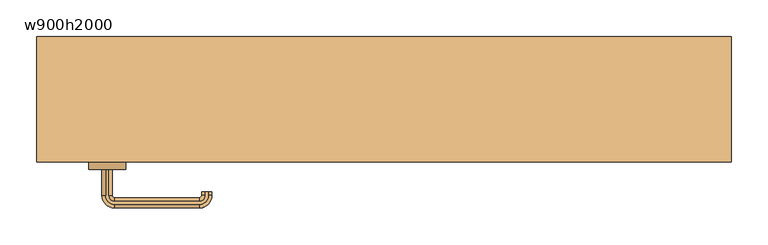
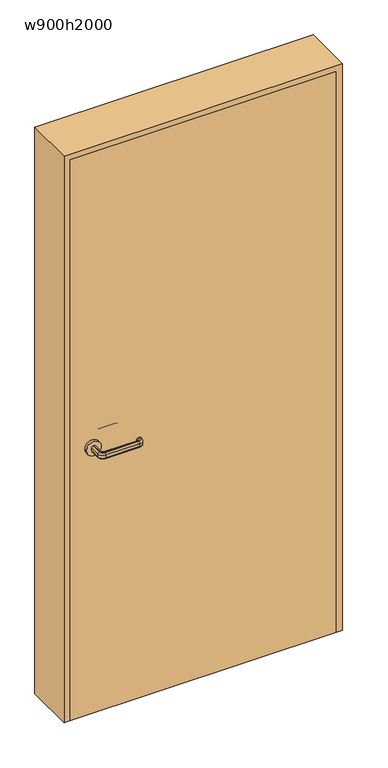
"""IFC4 building model written with IfcOpenShell, lengths in millimetres: door geometry, 片開き : w900h2000."""

from ifc_helpers import new_model, si_unit, point, frame, frame_2d, origin, origin_with_axes, place, context, project, spatial, polyline, circle_curve, ellipse_curve, trimmed, segment, composite_curve, outline, extrude, source, transform, mapped, element, save
from ifc_brep_helpers import plane_surface, cylinder_surface, revolved_surface, advanced_brep


def w900h2000_c063673d(model_context):
    return source(origin(), model_context, "Body", "SolidModel", [
        advanced_brep(
        [(-377.0, -95.0, 960.0), (-373.0, -95.0, 960.0), (-368.0, -95.0, 955.0), (-368.0, -95.0, 945.0477623), (-373.0, -95.0, 940.0477623), (-377.0, -95.0, 940.0477623), (-382.0, -95.0, 945.0477623), (-382.0, -95.0, 955.0), (-382.0, -130.0, 955.0), (-377.0, -130.0, 960.0), (-382.0, -130.0, 945.0477623), (-377.0, -130.0, 940.0477623), (-373.0, -130.0, 940.0477623), (-365.0, -138.0, 940.0477623), (-250.0, -138.0, 940.0477623), (-242.0, -130.0, 940.0477623), (-242.0, -125.0, 940.0477623), (-238.0, -125.0, 940.0477623), (-238.0, -130.0, 940.0477623), (-250.0, -142.0, 940.0477623), (-365.0, -142.0, 940.0477623), (-368.0, -130.0, 945.0477623), (-368.0, -130.0, 955.0), (-373.0, -130.0, 960.0), (-365.0, -142.0, 960.0), (-250.0, -142.0, 960.0), (-238.0, -130.0, 960.0), (-238.0, -125.0, 960.0), (-242.0, -125.0, 960.0), (-242.0, -130.0, 960.0), (-250.0, -138.0, 960.0), (-365.0, -138.0, 960.0), (-365.0, -147.0, 955.0), (-365.0, -147.0, 945.0477623), (-365.0, -133.0, 945.0477623), (-365.0, -133.0, 955.0), (-250.0, -147.0, 955.0), (-250.0, -147.0, 945.0477623), (-250.0, -133.0, 945.0477623), (-250.0, -133.0, 955.0), (-233.0, -130.0, 955.0), (-233.0, -130.0, 945.0477623), (-247.0, -130.0, 945.0477623), (-247.0, -130.0, 955.0), (-233.0, -125.0, 955.0), (-233.0, -125.0, 945.0477623), (-247.0, -125.0, 945.0477623), (-247.0, -125.0, 955.0)],
        [
            (0, 1),
            (1, 2, circle_curve(frame((-373.0, -95.0, 955.0), z_axis=(0.0, 1.0, 0.0), x_axis=(-1.0, 0.0, 0.0)), 5.0)),
            (2, 3),
            (3, 4, circle_curve(frame((-373.0, -95.0, 945.0477623), z_axis=(0.0, 1.0, 0.0), x_axis=(-1.0, 0.0, 0.0)), 5.0)),
            (4, 5),
            (5, 6, circle_curve(frame((-377.0, -95.0, 945.0477623), z_axis=(0.0, 1.0, 0.0), x_axis=(-1.0, 0.0, 0.0)), 5.0)),
            (6, 7),
            (7, 0, circle_curve(frame((-377.0, -95.0, 955.0), z_axis=(0.0, 1.0, 0.0), x_axis=(-1.0, 0.0, 0.0)), 5.0)),
            (7, 8),
            (8, 9, circle_curve(frame((-377.0, -130.0, 955.0), z_axis=(0.0, 1.0, 0.0), x_axis=(-1.0, 0.0, 0.0)), 5.0)),
            (9, 0),
            (6, 10),
            (10, 8),
            (5, 11),
            (11, 10, circle_curve(frame((-377.0, -130.0, 945.0477623), z_axis=(0.0, 1.0, 0.0), x_axis=(-1.0, 0.0, 0.0)), 5.0)),
            (4, 12),
            (12, 13, circle_curve(frame((-365.0, -130.0, 940.0477623), z_axis=(0.0, 0.0, 1.0), x_axis=(-1.0, 0.0, 0.0)), 8.0)),
            (13, 14),
            (14, 15, circle_curve(frame((-250.0, -130.0, 940.0477623), z_axis=(0.0, 0.0, 1.0), x_axis=(0.0, -1.0, 0.0)), 8.0)),
            (15, 16),
            (16, 17),
            (17, 18),
            (18, 19, circle_curve(frame((-250.0, -130.0, 940.0477623), z_axis=(0.0, 0.0, -1.0), x_axis=(0.0, -1.0, 0.0)), 12.0)),
            (19, 20),
            (20, 11, circle_curve(frame((-365.0, -130.0, 940.0477623), z_axis=(0.0, 0.0, -1.0), x_axis=(-1.0, 0.0, 0.0)), 12.0)),
            (3, 21),
            (21, 12, circle_curve(frame((-373.0, -130.0, 945.0477623), z_axis=(0.0, 1.0, 0.0), x_axis=(-1.0, 0.0, 0.0)), 5.0)),
            (2, 22),
            (22, 21),
            (1, 23),
            (23, 22, circle_curve(frame((-373.0, -130.0, 955.0), z_axis=(0.0, 1.0, 0.0), x_axis=(-1.0, 0.0, 0.0)), 5.0)),
            (9, 24, circle_curve(frame((-365.0, -130.0, 960.0), z_axis=(0.0, 0.0, 1.0), x_axis=(-1.0, 0.0, 0.0)), 12.0)),
            (24, 25),
            (25, 26, circle_curve(frame((-250.0, -130.0, 960.0), z_axis=(0.0, 0.0, 1.0), x_axis=(0.0, -1.0, 0.0)), 12.0)),
            (26, 27),
            (27, 28),
            (28, 29),
            (29, 30, circle_curve(frame((-250.0, -130.0, 960.0), z_axis=(0.0, 0.0, -1.0), x_axis=(0.0, -1.0, 0.0)), 8.0)),
            (30, 31),
            (31, 23, circle_curve(frame((-365.0, -130.0, 960.0), z_axis=(0.0, 0.0, -1.0), x_axis=(-1.0, 0.0, 0.0)), 8.0)),
            (32, 24, circle_curve(frame((-365.0, -142.0, 955.0), z_axis=(-1.0, 0.0, 0.0), x_axis=(0.0, -1.0, 0.0)), 5.0)),
            (8, 32, circle_curve(frame((-365.0, -130.0, 955.0), z_axis=(0.0, 0.0, 1.0), x_axis=(-1.0, 0.0, 0.0)), 17.0)),
            (33, 32),
            (10, 33, circle_curve(frame((-365.0, -130.0, 945.0477623), z_axis=(0.0, 0.0, 1.0), x_axis=(-1.0, 0.0, 0.0)), 17.0)),
            (20, 33, circle_curve(frame((-365.0, -142.0, 945.0477623), z_axis=(-1.0, 0.0, 0.0), x_axis=(0.0, -1.0, 0.0)), 5.0)),
            (34, 13, circle_curve(frame((-365.0, -138.0, 945.0477623), z_axis=(-1.0, 0.0, 0.0), x_axis=(0.0, -1.0, 0.0)), 5.0)),
            (21, 34, circle_curve(frame((-365.0, -130.0, 945.0477623), z_axis=(0.0, 0.0, 1.0), x_axis=(-1.0, 0.0, 0.0)), 3.0)),
            (35, 34),
            (22, 35, circle_curve(frame((-365.0, -130.0, 955.0), z_axis=(0.0, 0.0, 1.0), x_axis=(-1.0, 0.0, 0.0)), 3.0)),
            (31, 35, circle_curve(frame((-365.0, -138.0, 955.0), z_axis=(-1.0, 0.0, 0.0), x_axis=(0.0, -1.0, 0.0)), 5.0)),
            (32, 36),
            (36, 25, circle_curve(frame((-250.0, -142.0, 955.0), z_axis=(-1.0, 0.0, 0.0), x_axis=(0.0, -1.0, 0.0)), 5.0)),
            (33, 37),
            (37, 36),
            (19, 37, circle_curve(frame((-250.0, -142.0, 945.0477623), z_axis=(-1.0, 0.0, 0.0), x_axis=(0.0, -1.0, 0.0)), 5.0)),
            (34, 38),
            (38, 14, circle_curve(frame((-250.0, -138.0, 945.0477623), z_axis=(-1.0, 0.0, 0.0), x_axis=(0.0, -1.0, 0.0)), 5.0)),
            (35, 39),
            (39, 38),
            (30, 39, circle_curve(frame((-250.0, -138.0, 955.0), z_axis=(-1.0, 0.0, 0.0), x_axis=(0.0, -1.0, 0.0)), 5.0)),
            (40, 26, circle_curve(frame((-238.0, -130.0, 955.0), z_axis=(0.0, -1.0, 0.0), x_axis=(1.0, 0.0, 0.0)), 5.0)),
            (36, 40, circle_curve(frame((-250.0, -130.0, 955.0), z_axis=(0.0, 0.0, 1.0), x_axis=(0.0, -1.0, 0.0)), 17.0)),
            (41, 40),
            (37, 41, circle_curve(frame((-250.0, -130.0, 945.0477623), z_axis=(0.0, 0.0, 1.0), x_axis=(0.0, -1.0, 0.0)), 17.0)),
            (18, 41, circle_curve(frame((-238.0, -130.0, 945.0477623), z_axis=(0.0, -1.0, 0.0), x_axis=(1.0, 0.0, 0.0)), 5.0)),
            (42, 15, circle_curve(frame((-242.0, -130.0, 945.0477623), z_axis=(0.0, -1.0, 0.0), x_axis=(1.0, 0.0, 0.0)), 5.0)),
            (38, 42, circle_curve(frame((-250.0, -130.0, 945.0477623), z_axis=(0.0, 0.0, 1.0), x_axis=(0.0, -1.0, 0.0)), 3.0)),
            (43, 42),
            (39, 43, circle_curve(frame((-250.0, -130.0, 955.0), z_axis=(0.0, 0.0, 1.0), x_axis=(0.0, -1.0, 0.0)), 3.0)),
            (29, 43, circle_curve(frame((-242.0, -130.0, 955.0), z_axis=(0.0, -1.0, 0.0), x_axis=(1.0, 0.0, 0.0)), 5.0)),
            (27, 44, circle_curve(frame((-238.0, -125.0, 955.0), z_axis=(0.0, 1.0, 0.0), x_axis=(1.0, 0.0, 0.0)), 5.0)),
            (44, 45),
            (45, 17, circle_curve(frame((-238.0, -125.0, 945.0477623), z_axis=(0.0, 1.0, 0.0), x_axis=(1.0, 0.0, 0.0)), 5.0)),
            (16, 46, circle_curve(frame((-242.0, -125.0, 945.0477623), z_axis=(0.0, 1.0, 0.0), x_axis=(1.0, 0.0, 0.0)), 5.0)),
            (46, 47),
            (47, 28, circle_curve(frame((-242.0, -125.0, 955.0), z_axis=(0.0, 1.0, 0.0), x_axis=(1.0, 0.0, 0.0)), 5.0)),
            (40, 44),
            (41, 45),
            (42, 46),
            (43, 47),
        ],
        [
            plane_surface(frame((-385.198039, -95.0, 950.0), z_axis=(0.0, 1.0, 0.0), x_axis=(0.0, 0.0, 1.0))),
            cylinder_surface(frame((-377.0, -95.0, 955.0), z_axis=(0.0, 1.0, 0.0), x_axis=(-1.0, 0.0, 0.0)), 5.0),
            plane_surface(frame((-382.0, -95.0, 955.0), z_axis=(-1.0, 0.0, 0.0), x_axis=(0.0, -1.0, 0.0))),
            cylinder_surface(frame((-377.0, -95.0, 945.0477623), z_axis=(0.0, 1.0, 0.0), x_axis=(-1.0, 0.0, 0.0)), 5.0),
            plane_surface(frame((-377.0, -95.0, 940.0477623), z_axis=(0.0, 0.0, -1.0), x_axis=(0.0, -1.0, 0.0))),
            cylinder_surface(frame((-373.0, -95.0, 945.0477623), z_axis=(0.0, 1.0, 0.0), x_axis=(-1.0, 0.0, 0.0)), 5.0),
            plane_surface(frame((-368.0, -95.0, 945.0477623), z_axis=(1.0, 0.0, 0.0), x_axis=(0.0, -1.0, 0.0))),
            cylinder_surface(frame((-373.0, -95.0, 955.0), z_axis=(0.0, 1.0, 0.0), x_axis=(-1.0, 0.0, 0.0)), 5.0),
            plane_surface(frame((-373.0, -95.0, 960.0), z_axis=(0.0, 0.0, 1.0), x_axis=(0.0, -1.0, 0.0))),
            revolved_surface(trimmed(ellipse_curve(frame((-377.0, -130.0, 955.0), z_axis=(0.0, -1.0, 0.0), x_axis=(-1.0, 0.0, 0.0)), 5.0, 5.0), [point((-377.0, -130.0, 960.0))], [point((-382.0, -130.0, 955.0))], True, "CARTESIAN"), (-365.0, -130.0, 950.0), (0.0, 0.0, -1.0)),
            cylinder_surface(frame((-365.0, -130.0, 950.0), z_axis=(0.0, 0.0, -1.0), x_axis=(-1.0, 0.0, 0.0)), 17.0),
            revolved_surface(trimmed(ellipse_curve(frame((-377.0, -130.0, 945.0477623), z_axis=(0.0, -1.0, 0.0), x_axis=(-1.0, 0.0, 0.0)), 5.0, 5.0), [point((-382.0, -130.0, 945.0477623))], [point((-377.0, -130.0, 940.0477623))], True, "CARTESIAN"), (-365.0, -130.0, 950.0), (0.0, 0.0, -1.0)),
            revolved_surface(trimmed(ellipse_curve(frame((-373.0, -130.0, 945.0477623), z_axis=(0.0, -1.0, 0.0), x_axis=(-1.0, 0.0, 0.0)), 5.0, 5.0), [point((-373.0, -130.0, 940.0477623))], [point((-368.0, -130.0, 945.0477623))], True, "CARTESIAN"), (-365.0, -130.0, 950.0), (0.0, 0.0, -1.0)),
            revolved_surface(polyline([(-368.0, -130.0, 945.0477623), (-368.0, -130.0, 955.0)]), (-365.0, -130.0, 950.0), (0.0, 0.0, -1.0)),
            revolved_surface(trimmed(ellipse_curve(frame((-373.0, -130.0, 955.0), z_axis=(0.0, -1.0, 0.0), x_axis=(-1.0, 0.0, 0.0)), 5.0, 5.0), [point((-368.0, -130.0, 955.0))], [point((-373.0, -130.0, 960.0))], True, "CARTESIAN"), (-365.0, -130.0, 950.0), (0.0, 0.0, -1.0)),
            cylinder_surface(frame((-365.0, -142.0, 955.0), z_axis=(-1.0, 0.0, 0.0), x_axis=(0.0, -1.0, 0.0)), 5.0),
            plane_surface(frame((-365.0, -147.0, 955.0), z_axis=(0.0, -1.0, 0.0), x_axis=(1.0, 0.0, 0.0))),
            cylinder_surface(frame((-365.0, -142.0, 945.0477623), z_axis=(-1.0, 0.0, 0.0), x_axis=(0.0, -1.0, 0.0)), 5.0),
            cylinder_surface(frame((-365.0, -138.0, 945.0477623), z_axis=(-1.0, 0.0, 0.0), x_axis=(0.0, -1.0, 0.0)), 5.0),
            plane_surface(frame((-365.0, -133.0, 945.0477623), z_axis=(0.0, 1.0, 0.0), x_axis=(1.0, 0.0, 0.0))),
            cylinder_surface(frame((-365.0, -138.0, 955.0), z_axis=(-1.0, 0.0, 0.0), x_axis=(0.0, -1.0, 0.0)), 5.0),
            revolved_surface(trimmed(ellipse_curve(frame((-250.0, -142.0, 955.0), z_axis=(1.0, 0.0, 0.0), x_axis=(0.0, -1.0, 0.0)), 5.0, 5.0), [point((-250.0, -142.0, 960.0))], [point((-250.0, -147.0, 955.0))], True, "CARTESIAN"), (-250.0, -130.0, 950.0), (0.0, 0.0, -1.0)),
            cylinder_surface(frame((-250.0, -130.0, 950.0), z_axis=(0.0, 0.0, -1.0), x_axis=(0.0, -1.0, 0.0)), 17.0),
            revolved_surface(trimmed(ellipse_curve(frame((-250.0, -142.0, 945.0477623), z_axis=(1.0, 0.0, 0.0), x_axis=(0.0, -1.0, 0.0)), 5.0, 5.0), [point((-250.0, -147.0, 945.0477623))], [point((-250.0, -142.0, 940.0477623))], True, "CARTESIAN"), (-250.0, -130.0, 950.0), (0.0, 0.0, -1.0)),
            revolved_surface(trimmed(ellipse_curve(frame((-250.0, -138.0, 945.0477623), z_axis=(1.0, 0.0, 0.0), x_axis=(0.0, -1.0, 0.0)), 5.0, 5.0), [point((-250.0, -138.0, 940.0477623))], [point((-250.0, -133.0, 945.0477623))], True, "CARTESIAN"), (-250.0, -130.0, 950.0), (0.0, 0.0, -1.0)),
            revolved_surface(polyline([(-250.0, -133.0, 945.0477623), (-250.0, -133.0, 955.0)]), (-250.0, -130.0, 950.0), (0.0, 0.0, -1.0)),
            revolved_surface(trimmed(ellipse_curve(frame((-250.0, -138.0, 955.0), z_axis=(1.0, 0.0, 0.0), x_axis=(0.0, -1.0, 0.0)), 5.0, 5.0), [point((-250.0, -133.0, 955.0))], [point((-250.0, -138.0, 960.0))], True, "CARTESIAN"), (-250.0, -130.0, 950.0), (0.0, 0.0, -1.0)),
            plane_surface(frame((-250.198039, -125.0, 950.0), z_axis=(0.0, 1.0, 0.0), x_axis=(0.0, 0.0, -1.0))),
            cylinder_surface(frame((-238.0, -130.0, 955.0), z_axis=(0.0, -1.0, 0.0), x_axis=(1.0, 0.0, 0.0)), 5.0),
            plane_surface(frame((-233.0, -130.0, 955.0), z_axis=(1.0, 0.0, 0.0), x_axis=(0.0, 1.0, 0.0))),
            cylinder_surface(frame((-238.0, -130.0, 945.0477623), z_axis=(0.0, -1.0, 0.0), x_axis=(1.0, 0.0, 0.0)), 5.0),
            cylinder_surface(frame((-242.0, -130.0, 945.0477623), z_axis=(0.0, -1.0, 0.0), x_axis=(1.0, 0.0, 0.0)), 5.0),
            plane_surface(frame((-247.0, -130.0, 945.0477623), z_axis=(-1.0, 0.0, 0.0), x_axis=(0.0, 1.0, 0.0))),
            cylinder_surface(frame((-242.0, -130.0, 955.0), z_axis=(0.0, -1.0, 0.0), x_axis=(1.0, 0.0, 0.0)), 5.0),
        ],
        [
            (0, [[1, 2, 3, 4, 5, 6, 7, 8]]),
            (1, [[9, 10, 11, -8]]),
            (2, [[12, 13, -9, -7]]),
            (3, [[14, 15, -12, -6]]),
            (4, [[16, 17, 18, 19, 20, 21, 22, 23, 24, 25, -14, -5]]),
            (5, [[26, 27, -16, -4]]),
            (6, [[28, 29, -26, -3]]),
            (7, [[30, 31, -28, -2]]),
            (8, [[-11, 32, 33, 34, 35, 36, 37, 38, 39, 40, -30, -1]]),
            (9, [[41, -32, -10, 42]]),
            (10, [[43, -42, -13, 44]]),
            (11, [[45, -44, -15, -25]]),
            (12, [[46, -17, -27, 47]]),
            (13, [[48, -47, -29, 49]]),
            (14, [[50, -49, -31, -40]]),
            (15, [[51, 52, -33, -41]]),
            (16, [[53, 54, -51, -43]]),
            (17, [[-24, 55, -53, -45]]),
            (18, [[56, 57, -18, -46]]),
            (19, [[58, 59, -56, -48]]),
            (20, [[-39, 60, -58, -50]]),
            (21, [[61, -34, -52, 62]]),
            (22, [[63, -62, -54, 64]]),
            (23, [[65, -64, -55, -23]]),
            (24, [[66, -19, -57, 67]]),
            (25, [[68, -67, -59, 69]]),
            (26, [[70, -69, -60, -38]]),
            (27, [[71, 72, 73, -21, 74, 75, 76, -36]]),
            (28, [[77, -71, -35, -61]]),
            (29, [[78, -72, -77, -63]]),
            (30, [[-22, -73, -78, -65]]),
            (31, [[79, -74, -20, -66]]),
            (32, [[80, -75, -79, -68]]),
            (33, [[-37, -76, -80, -70]]),
        ],
    ),
        advanced_brep(
        [(-373.0, -45.0, 940.0), (-368.0, -45.0, 945.0), (-368.0, -45.0, 955.0), (-373.0, -45.0, 960.0), (-377.0, -45.0, 960.0), (-382.0, -45.0, 955.0), (-382.0, -45.0, 945.0), (-377.0, -45.0, 940.0), (-377.0, -10.0, 940.0), (-365.0, 2.0, 940.0), (-250.0, 2.0, 940.0), (-238.0, -10.0, 940.0), (-238.0, -15.0, 940.0), (-242.0, -15.0, 940.0), (-242.0, -10.0, 940.0), (-250.0, -2.0, 940.0), (-365.0, -2.0, 940.0), (-373.0, -10.0, 940.0), (-382.0, -10.0, 945.0), (-382.0, -10.0, 955.0), (-377.0, -10.0, 960.0), (-373.0, -10.0, 960.0), (-365.0, -2.0, 960.0), (-250.0, -2.0, 960.0), (-242.0, -10.0, 960.0), (-242.0, -15.0, 960.0), (-238.0, -15.0, 960.0), (-238.0, -10.0, 960.0), (-250.0, 2.0, 960.0), (-365.0, 2.0, 960.0), (-368.0, -10.0, 955.0), (-368.0, -10.0, 945.0), (-365.0, 7.0, 945.0), (-365.0, 7.0, 955.0), (-365.0, -7.0, 955.0), (-365.0, -7.0, 945.0), (-250.0, 7.0, 945.0), (-250.0, 7.0, 955.0), (-250.0, -7.0, 955.0), (-250.0, -7.0, 945.0), (-233.0, -10.0, 945.0), (-233.0, -10.0, 955.0), (-247.0, -10.0, 955.0), (-247.0, -10.0, 945.0), (-233.0, -15.0, 945.0), (-233.0, -15.0, 955.0), (-247.0, -15.0, 955.0), (-247.0, -15.0, 945.0)],
        [
            (0, 1, circle_curve(frame((-373.0, -45.0, 945.0), z_axis=(0.0, -1.0, 0.0), x_axis=(1.0, 0.0, 0.0)), 5.0)),
            (1, 2),
            (2, 3, circle_curve(frame((-373.0, -45.0, 955.0), z_axis=(0.0, -1.0, 0.0), x_axis=(1.0, 0.0, 0.0)), 5.0)),
            (3, 4),
            (4, 5, circle_curve(frame((-377.0, -45.0, 955.0), z_axis=(0.0, -1.0, 0.0), x_axis=(1.0, 0.0, 0.0)), 5.0)),
            (5, 6),
            (6, 7, circle_curve(frame((-377.0, -45.0, 945.0), z_axis=(0.0, -1.0, 0.0), x_axis=(1.0, 0.0, 0.0)), 5.0)),
            (7, 0),
            (7, 8),
            (8, 9, circle_curve(frame((-365.0, -10.0, 940.0), z_axis=(0.0, 0.0, -1.0), x_axis=(-1.0, 0.0, 0.0)), 12.0)),
            (9, 10),
            (10, 11, circle_curve(frame((-250.0, -10.0, 940.0), z_axis=(0.0, 0.0, -1.0), x_axis=(0.0, 1.0, 0.0)), 12.0)),
            (11, 12),
            (12, 13),
            (13, 14),
            (14, 15, circle_curve(frame((-250.0, -10.0, 940.0), z_axis=(0.0, 0.0, 1.0), x_axis=(0.0, 1.0, 0.0)), 8.0)),
            (15, 16),
            (16, 17, circle_curve(frame((-365.0, -10.0, 940.0), z_axis=(0.0, 0.0, 1.0), x_axis=(-1.0, 0.0, 0.0)), 8.0)),
            (17, 0),
            (6, 18),
            (18, 8, circle_curve(frame((-377.0, -10.0, 945.0), z_axis=(0.0, -1.0, 0.0), x_axis=(1.0, 0.0, 0.0)), 5.0)),
            (5, 19),
            (19, 18),
            (4, 20),
            (20, 19, circle_curve(frame((-377.0, -10.0, 955.0), z_axis=(0.0, -1.0, 0.0), x_axis=(1.0, 0.0, 0.0)), 5.0)),
            (3, 21),
            (21, 22, circle_curve(frame((-365.0, -10.0, 960.0), z_axis=(0.0, 0.0, -1.0), x_axis=(-1.0, 0.0, 0.0)), 8.0)),
            (22, 23),
            (23, 24, circle_curve(frame((-250.0, -10.0, 960.0), z_axis=(0.0, 0.0, -1.0), x_axis=(0.0, 1.0, 0.0)), 8.0)),
            (24, 25),
            (25, 26),
            (26, 27),
            (27, 28, circle_curve(frame((-250.0, -10.0, 960.0), z_axis=(0.0, 0.0, 1.0), x_axis=(0.0, 1.0, 0.0)), 12.0)),
            (28, 29),
            (29, 20, circle_curve(frame((-365.0, -10.0, 960.0), z_axis=(0.0, 0.0, 1.0), x_axis=(-1.0, 0.0, 0.0)), 12.0)),
            (2, 30),
            (30, 21, circle_curve(frame((-373.0, -10.0, 955.0), z_axis=(0.0, -1.0, 0.0), x_axis=(1.0, 0.0, 0.0)), 5.0)),
            (1, 31),
            (31, 30),
            (17, 31, circle_curve(frame((-373.0, -10.0, 945.0), z_axis=(0.0, -1.0, 0.0), x_axis=(1.0, 0.0, 0.0)), 5.0)),
            (32, 9, circle_curve(frame((-365.0, 2.0, 945.0), z_axis=(-1.0, 0.0, 0.0), x_axis=(0.0, -1.0, 0.0)), 5.0)),
            (18, 32, circle_curve(frame((-365.0, -10.0, 945.0), z_axis=(0.0, 0.0, -1.0), x_axis=(-1.0, 0.0, 0.0)), 17.0)),
            (33, 32),
            (19, 33, circle_curve(frame((-365.0, -10.0, 955.0), z_axis=(0.0, 0.0, -1.0), x_axis=(-1.0, 0.0, 0.0)), 17.0)),
            (29, 33, circle_curve(frame((-365.0, 2.0, 955.0), z_axis=(-1.0, 0.0, 0.0), x_axis=(0.0, -1.0, 0.0)), 5.0)),
            (34, 22, circle_curve(frame((-365.0, -2.0, 955.0), z_axis=(-1.0, 0.0, 0.0), x_axis=(0.0, -1.0, 0.0)), 5.0)),
            (30, 34, circle_curve(frame((-365.0, -10.0, 955.0), z_axis=(0.0, 0.0, -1.0), x_axis=(-1.0, 0.0, 0.0)), 3.0)),
            (35, 34),
            (31, 35, circle_curve(frame((-365.0, -10.0, 945.0), z_axis=(0.0, 0.0, -1.0), x_axis=(-1.0, 0.0, 0.0)), 3.0)),
            (16, 35, circle_curve(frame((-365.0, -2.0, 945.0), z_axis=(-1.0, 0.0, 0.0), x_axis=(0.0, -1.0, 0.0)), 5.0)),
            (32, 36),
            (36, 10, circle_curve(frame((-250.0, 2.0, 945.0), z_axis=(-1.0, 0.0, 0.0), x_axis=(0.0, -1.0, 0.0)), 5.0)),
            (33, 37),
            (37, 36),
            (28, 37, circle_curve(frame((-250.0, 2.0, 955.0), z_axis=(-1.0, 0.0, 0.0), x_axis=(0.0, -1.0, 0.0)), 5.0)),
            (34, 38),
            (38, 23, circle_curve(frame((-250.0, -2.0, 955.0), z_axis=(-1.0, 0.0, 0.0), x_axis=(0.0, -1.0, 0.0)), 5.0)),
            (35, 39),
            (39, 38),
            (15, 39, circle_curve(frame((-250.0, -2.0, 945.0), z_axis=(-1.0, 0.0, 0.0), x_axis=(0.0, -1.0, 0.0)), 5.0)),
            (40, 11, circle_curve(frame((-238.0, -10.0, 945.0), z_axis=(0.0, 1.0, 0.0), x_axis=(-1.0, 0.0, 0.0)), 5.0)),
            (36, 40, circle_curve(frame((-250.0, -10.0, 945.0), z_axis=(0.0, 0.0, -1.0), x_axis=(0.0, 1.0, 0.0)), 17.0)),
            (41, 40),
            (37, 41, circle_curve(frame((-250.0, -10.0, 955.0), z_axis=(0.0, 0.0, -1.0), x_axis=(0.0, 1.0, 0.0)), 17.0)),
            (27, 41, circle_curve(frame((-238.0, -10.0, 955.0), z_axis=(0.0, 1.0, 0.0), x_axis=(-1.0, 0.0, 0.0)), 5.0)),
            (42, 24, circle_curve(frame((-242.0, -10.0, 955.0), z_axis=(0.0, 1.0, 0.0), x_axis=(-1.0, 0.0, 0.0)), 5.0)),
            (38, 42, circle_curve(frame((-250.0, -10.0, 955.0), z_axis=(0.0, 0.0, -1.0), x_axis=(0.0, 1.0, 0.0)), 3.0)),
            (43, 42),
            (39, 43, circle_curve(frame((-250.0, -10.0, 945.0), z_axis=(0.0, 0.0, -1.0), x_axis=(0.0, 1.0, 0.0)), 3.0)),
            (14, 43, circle_curve(frame((-242.0, -10.0, 945.0), z_axis=(0.0, 1.0, 0.0), x_axis=(-1.0, 0.0, 0.0)), 5.0)),
            (12, 44, circle_curve(frame((-238.0, -15.0, 945.0), z_axis=(0.0, -1.0, 0.0), x_axis=(-1.0, 0.0, 0.0)), 5.0)),
            (44, 45),
            (45, 26, circle_curve(frame((-238.0, -15.0, 955.0), z_axis=(0.0, -1.0, 0.0), x_axis=(-1.0, 0.0, 0.0)), 5.0)),
            (25, 46, circle_curve(frame((-242.0, -15.0, 955.0), z_axis=(0.0, -1.0, 0.0), x_axis=(-1.0, 0.0, 0.0)), 5.0)),
            (46, 47),
            (47, 13, circle_curve(frame((-242.0, -15.0, 945.0), z_axis=(0.0, -1.0, 0.0), x_axis=(-1.0, 0.0, 0.0)), 5.0)),
            (40, 44),
            (41, 45),
            (42, 46),
            (43, 47),
        ],
        [
            plane_surface(frame((-385.198039, -45.0, 950.0), z_axis=(0.0, -1.0, 0.0), x_axis=(0.0, 0.0, -1.0))),
            plane_surface(frame((-373.0, -45.0, 940.0), z_axis=(0.0, 0.0, -1.0), x_axis=(0.0, 1.0, 0.0))),
            cylinder_surface(frame((-377.0, -45.0, 945.0), z_axis=(0.0, -1.0, 0.0), x_axis=(1.0, 0.0, 0.0)), 5.0),
            plane_surface(frame((-382.0, -45.0, 945.0), z_axis=(-1.0, 0.0, 0.0), x_axis=(0.0, 1.0, 0.0))),
            cylinder_surface(frame((-377.0, -45.0, 955.0), z_axis=(0.0, -1.0, 0.0), x_axis=(1.0, 0.0, 0.0)), 5.0),
            plane_surface(frame((-377.0, -45.0, 960.0), z_axis=(0.0, 0.0, 1.0), x_axis=(0.0, 1.0, 0.0))),
            cylinder_surface(frame((-373.0, -45.0, 955.0), z_axis=(0.0, -1.0, 0.0), x_axis=(1.0, 0.0, 0.0)), 5.0),
            plane_surface(frame((-368.0, -45.0, 955.0), z_axis=(1.0, 0.0, 0.0), x_axis=(0.0, 1.0, 0.0))),
            cylinder_surface(frame((-373.0, -45.0, 945.0), z_axis=(0.0, -1.0, 0.0), x_axis=(1.0, 0.0, 0.0)), 5.0),
            revolved_surface(trimmed(ellipse_curve(frame((-377.0, -10.0, 945.0), z_axis=(0.0, 1.0, 0.0), x_axis=(1.0, 0.0, 0.0)), 5.0, 5.0), [point((-377.0, -10.0, 940.0))], [point((-382.0, -10.0, 945.0))], True, "CARTESIAN"), (-365.0, -10.0, 950.0), (0.0, 0.0, 1.0)),
            cylinder_surface(frame((-365.0, -10.0, 950.0), z_axis=(0.0, 0.0, 1.0), x_axis=(-1.0, 0.0, 0.0)), 17.0),
            revolved_surface(trimmed(ellipse_curve(frame((-377.0, -10.0, 955.0), z_axis=(0.0, 1.0, 0.0), x_axis=(1.0, 0.0, 0.0)), 5.0, 5.0), [point((-382.0, -10.0, 955.0))], [point((-377.0, -10.0, 960.0))], True, "CARTESIAN"), (-365.0, -10.0, 950.0), (0.0, 0.0, 1.0)),
            revolved_surface(trimmed(ellipse_curve(frame((-373.0, -10.0, 955.0), z_axis=(0.0, 1.0, 0.0), x_axis=(1.0, 0.0, 0.0)), 5.0, 5.0), [point((-373.0, -10.0, 960.0))], [point((-368.0, -10.0, 955.0))], True, "CARTESIAN"), (-365.0, -10.0, 950.0), (0.0, 0.0, 1.0)),
            revolved_surface(polyline([(-368.0, -10.0, 955.0), (-368.0, -10.0, 945.0)]), (-365.0, -10.0, 950.0), (0.0, 0.0, 1.0)),
            revolved_surface(trimmed(ellipse_curve(frame((-373.0, -10.0, 945.0), z_axis=(0.0, 1.0, 0.0), x_axis=(1.0, 0.0, 0.0)), 5.0, 5.0), [point((-368.0, -10.0, 945.0))], [point((-373.0, -10.0, 940.0))], True, "CARTESIAN"), (-365.0, -10.0, 950.0), (0.0, 0.0, 1.0)),
            cylinder_surface(frame((-365.0, 2.0, 945.0), z_axis=(-1.0, 0.0, 0.0), x_axis=(0.0, -1.0, 0.0)), 5.0),
            plane_surface(frame((-365.0, 7.0, 945.0), z_axis=(0.0, 1.0, 0.0), x_axis=(1.0, 0.0, 0.0))),
            cylinder_surface(frame((-365.0, 2.0, 955.0), z_axis=(-1.0, 0.0, 0.0), x_axis=(0.0, -1.0, 0.0)), 5.0),
            cylinder_surface(frame((-365.0, -2.0, 955.0), z_axis=(-1.0, 0.0, 0.0), x_axis=(0.0, -1.0, 0.0)), 5.0),
            plane_surface(frame((-365.0, -7.0, 955.0), z_axis=(0.0, -1.0, 0.0), x_axis=(1.0, 0.0, 0.0))),
            cylinder_surface(frame((-365.0, -2.0, 945.0), z_axis=(-1.0, 0.0, 0.0), x_axis=(0.0, -1.0, 0.0)), 5.0),
            revolved_surface(trimmed(ellipse_curve(frame((-250.0, 2.0, 945.0), z_axis=(1.0, 0.0, 0.0), x_axis=(0.0, -1.0, 0.0)), 5.0, 5.0), [point((-250.0, 2.0, 940.0))], [point((-250.0, 7.0, 945.0))], True, "CARTESIAN"), (-250.0, -10.0, 950.0), (0.0, 0.0, 1.0)),
            cylinder_surface(frame((-250.0, -10.0, 950.0), z_axis=(0.0, 0.0, 1.0), x_axis=(0.0, 1.0, 0.0)), 17.0),
            revolved_surface(trimmed(ellipse_curve(frame((-250.0, 2.0, 955.0), z_axis=(1.0, 0.0, 0.0), x_axis=(0.0, -1.0, 0.0)), 5.0, 5.0), [point((-250.0, 7.0, 955.0))], [point((-250.0, 2.0, 960.0))], True, "CARTESIAN"), (-250.0, -10.0, 950.0), (0.0, 0.0, 1.0)),
            revolved_surface(trimmed(ellipse_curve(frame((-250.0, -2.0, 955.0), z_axis=(1.0, 0.0, 0.0), x_axis=(0.0, -1.0, 0.0)), 5.0, 5.0), [point((-250.0, -2.0, 960.0))], [point((-250.0, -7.0, 955.0))], True, "CARTESIAN"), (-250.0, -10.0, 950.0), (0.0, 0.0, 1.0)),
            revolved_surface(polyline([(-250.0, -7.0, 955.0), (-250.0, -7.0, 945.0)]), (-250.0, -10.0, 950.0), (0.0, 0.0, 1.0)),
            revolved_surface(trimmed(ellipse_curve(frame((-250.0, -2.0, 945.0), z_axis=(1.0, 0.0, 0.0), x_axis=(0.0, -1.0, 0.0)), 5.0, 5.0), [point((-250.0, -7.0, 945.0))], [point((-250.0, -2.0, 940.0))], True, "CARTESIAN"), (-250.0, -10.0, 950.0), (0.0, 0.0, 1.0)),
            plane_surface(frame((-250.198039, -15.0, 950.0), z_axis=(0.0, -1.0, 0.0), x_axis=(0.0, 0.0, 1.0))),
            cylinder_surface(frame((-238.0, -10.0, 945.0), z_axis=(0.0, 1.0, 0.0), x_axis=(-1.0, 0.0, 0.0)), 5.0),
            plane_surface(frame((-233.0, -10.0, 945.0), z_axis=(1.0, 0.0, 0.0), x_axis=(0.0, -1.0, 0.0))),
            cylinder_surface(frame((-238.0, -10.0, 955.0), z_axis=(0.0, 1.0, 0.0), x_axis=(-1.0, 0.0, 0.0)), 5.0),
            cylinder_surface(frame((-242.0, -10.0, 955.0), z_axis=(0.0, 1.0, 0.0), x_axis=(-1.0, 0.0, 0.0)), 5.0),
            plane_surface(frame((-247.0, -10.0, 955.0), z_axis=(-1.0, 0.0, 0.0), x_axis=(0.0, -1.0, 0.0))),
            cylinder_surface(frame((-242.0, -10.0, 945.0), z_axis=(0.0, 1.0, 0.0), x_axis=(-1.0, 0.0, 0.0)), 5.0),
        ],
        [
            (0, [[1, 2, 3, 4, 5, 6, 7, 8]]),
            (1, [[9, 10, 11, 12, 13, 14, 15, 16, 17, 18, 19, -8]]),
            (2, [[20, 21, -9, -7]]),
            (3, [[22, 23, -20, -6]]),
            (4, [[24, 25, -22, -5]]),
            (5, [[26, 27, 28, 29, 30, 31, 32, 33, 34, 35, -24, -4]]),
            (6, [[36, 37, -26, -3]]),
            (7, [[38, 39, -36, -2]]),
            (8, [[-19, 40, -38, -1]]),
            (9, [[41, -10, -21, 42]]),
            (10, [[43, -42, -23, 44]]),
            (11, [[45, -44, -25, -35]]),
            (12, [[46, -27, -37, 47]]),
            (13, [[48, -47, -39, 49]]),
            (14, [[50, -49, -40, -18]]),
            (15, [[51, 52, -11, -41]]),
            (16, [[53, 54, -51, -43]]),
            (17, [[-34, 55, -53, -45]]),
            (18, [[56, 57, -28, -46]]),
            (19, [[58, 59, -56, -48]]),
            (20, [[-17, 60, -58, -50]]),
            (21, [[61, -12, -52, 62]]),
            (22, [[63, -62, -54, 64]]),
            (23, [[65, -64, -55, -33]]),
            (24, [[66, -29, -57, 67]]),
            (25, [[68, -67, -59, 69]]),
            (26, [[70, -69, -60, -16]]),
            (27, [[-14, 71, 72, 73, -31, 74, 75, 76]]),
            (28, [[77, -71, -13, -61]]),
            (29, [[78, -72, -77, -63]]),
            (30, [[-32, -73, -78, -65]]),
            (31, [[79, -74, -30, -66]]),
            (32, [[80, -75, -79, -68]]),
            (33, [[-15, -76, -80, -70]]),
        ],
    ),
        extrude(outline(composite_curve([segment(trimmed(circle_curve(frame_2d((950.0, -375.0)), 25.0), [point((950.0, -400.0))], [point((950.0, -350.0))], False, "CARTESIAN"), True, "CONTINUOUS"), segment(trimmed(circle_curve(frame_2d((950.0, -375.0)), 25.0), [point((950.0, -350.0))], [point((950.0, -400.0))], False, "CARTESIAN"), True, "CONTINUOUS")], self_intersect=False)), frame((0.0, -95.0, 0.0), z_axis=(0.0, 1.0, 0.0), x_axis=(0.0, 0.0, 1.0)), (0.0, 0.0, 1.0), 10.0),
        extrude(outline(composite_curve([segment(trimmed(circle_curve(frame_2d((950.0, -375.0)), 25.0), [point((950.0, -400.0))], [point((950.0, -350.0))], False, "CARTESIAN"), True, "CONTINUOUS"), segment(trimmed(circle_curve(frame_2d((950.0, -375.0)), 25.0), [point((950.0, -350.0))], [point((950.0, -400.0))], False, "CARTESIAN"), True, "CONTINUOUS")], self_intersect=False)), frame((0.0, -55.0, 0.0), z_axis=(0.0, 1.0, 0.0), x_axis=(0.0, 0.0, 1.0)), (0.0, 0.0, 1.0), 10.0),
        extrude(outline(polyline([(2020.0, -470.0), (0.0, -470.0), (0.0, -450.0), (2000.0, -450.0), (2000.0, 450.0), (0.0, 450.0), (0.0, 470.0), (2020.0, 470.0), (2020.0, -470.0)])), frame((0.0, -85.0, 0.0), z_axis=(0.0, 1.0, 0.0), x_axis=(0.0, 0.0, 1.0)), (0.0, 0.0, 1.0), 170.0),
        extrude(outline(polyline([(450.0, -55.0), (450.0, -85.0), (-450.0, -85.0), (-450.0, -55.0), (450.0, -55.0)])), origin_with_axes(), (0.0, 0.0, 1.0), 2000.0),
    ])


if __name__ == "__main__":
    model = new_model("IFC4")
    model_context = context("Model", 3, world=origin())
    ifc_project = project(units=[si_unit("LENGTHUNIT", "METRE", prefix="MILLI")], contexts=[model_context])
    site = spatial("IfcSite", under=ifc_project)
    building = spatial("IfcBuilding", under=site)
    placement = place(None, origin())
    w900h2000_shape = w900h2000_c063673d(model_context)
    element("IfcDoor", 1, ObjectType="片開き : w900h2000", at=placement, inside=building, context=model_context, shape_type="MappedRepresentation", body=[
        mapped(w900h2000_shape, transform((0.0, 0.0, 0.0), x_axis=(1.0, 0.0, 0.0), y_axis=(0.0, 1.0, 0.0), z_axis=(0.0, 0.0, 1.0))),
    ])
    save(model, "model.ifc")

# Revit data of these elements
# Type "片開き : w900h2000"
#   Construction Type Id = "MDOOR"
#   Analytic Construction = "メタル"
#   Type Mark = "48"
#   Operation = "片側開き戸右"
#   Keynote = "08110.P2"
#   Visual Light Transmittance = 0
#   Solar Heat Gain Coefficient = 0
#   Heat Transfer Coefficient (U) = 3.7021 W/(m²·K)
#   高さ(中心) = 1000 mm
#   Height = 2000 mm
#   Thickness = 30 mm
#   ドア枠見附 = 20 mm
#   Width = 900 mm
#   取手取付け高さ = 950 mm
#   ドア枠ちり = 10 mm
#   Function = 0
#   ドア枠 [instance default] = 塗装ホワイト
#   ドア把手 [instance default] = メタル-ステンレス
#   ドア [instance default] = 塗装ホワイト
#   Wall Closure = (empty or 0)
# Element 1 (IfcDoor, "片開き : w900h2000")
#   Materials on its faces: "メタル-ステンレス", "塗装ホワイト"
# Materials
#   "塗装ホワイト": class "ペイント", colour RGB 249 249 249, transparency 0, Cost = 0
#   "メタル-ステンレス": class "メタル", colour RGB 247 247 247, transparency 0, Cost = 0
